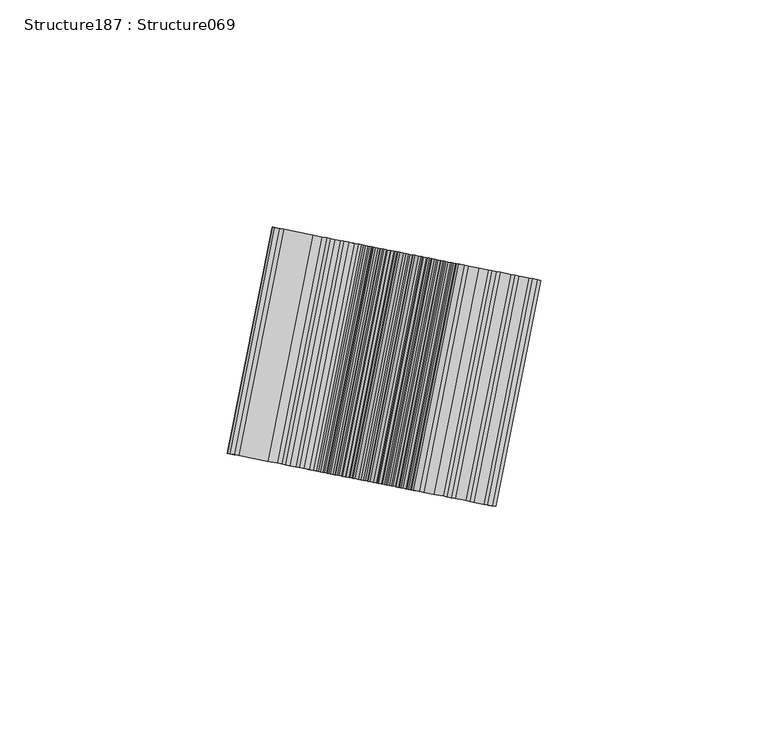
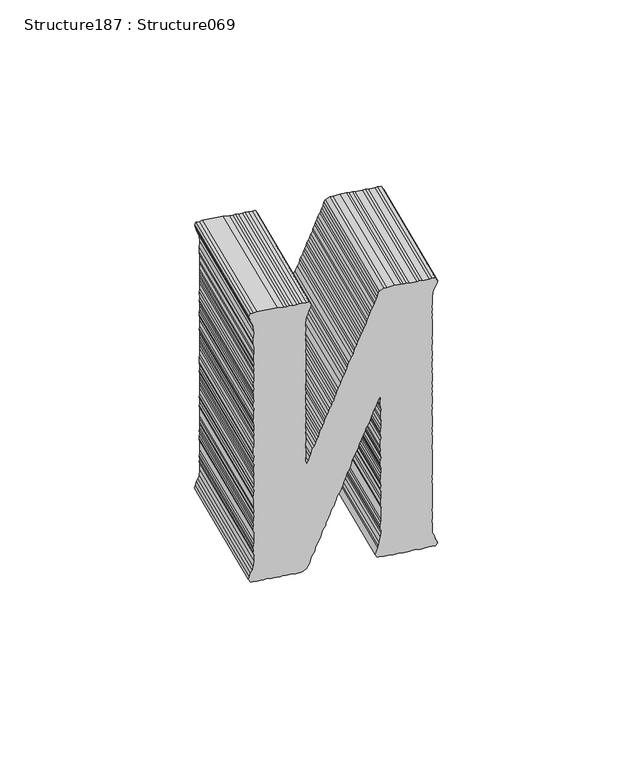
"""IFC4 building model written with IfcOpenShell, lengths in millimetres: proxy geometry, Structure187 : Structure069."""

import ifcopenshell
import ifcopenshell.guid

model = None  # the IFC model being written
_history = None  # IfcOwnerHistory: only IFC2X3 demands one
_inside = {}  # id of a spatial element -> (the spatial element, [elements in it])
_under = {}  # id of a project, library or spatial element -> (it, [spatial elements below it])
_declared = {}  # id of a project -> (the project, [libraries it declares])
_typed = {}  # id of a type object -> (the type object, [elements of that type])
_made_of = {}  # id of a material, layer set ... -> (it, [elements and type objects made of it])


def new_model(schema):
    """Start an empty IFC model of exactly this schema.

    Asked for "IFC4X3", IfcOpenShell would pick the latest addendum, in which some entities
    have other attributes; the version numbers below select the first issue.
    IFC2X3 requires an IfcOwnerHistory on every rooted entity: one is made here for all.
    """
    global model, _history
    if schema == "IFC4X3":
        model = ifcopenshell.file(schema_version=(4, 3, 0, 0))
    else:
        model = ifcopenshell.file(schema=schema)
    _inside.clear()
    _under.clear()
    _declared.clear()
    _typed.clear()
    _made_of.clear()
    _history = None
    if model.schema == "IFC2X3":
        org = make("IfcOrganization", Name="unknown")
        user = make(
            "IfcPersonAndOrganization",
            ThePerson=make("IfcPerson", FamilyName="unknown"),
            TheOrganization=org,
        )
        app = make(
            "IfcApplication",
            ApplicationDeveloper=org,
            Version="unknown",
            ApplicationFullName="unknown",
            ApplicationIdentifier="unknown",
        )
        _history = make(
            "IfcOwnerHistory",
            OwningUser=user,
            OwningApplication=app,
            ChangeAction="ADDED",
            CreationDate=0,
        )
    return model


def make(cls, **values):
    """One entity of the class cls with the attributes given. An attribute that is None is left unset."""
    return model.create_entity(
        cls, **{name: value for name, value in values.items() if value is not None}
    )


def rooted(cls, **values):
    """An entity with a GlobalId (a new one), such as an element, a storey or a relation."""
    return make(cls, GlobalId=ifcopenshell.guid.new(), OwnerHistory=_history, **values)


def si_unit(unit_type, name, prefix=None):
    """IfcSIUnit, for example si_unit("LENGTHUNIT", "METRE", prefix="MILLI")."""
    return make("IfcSIUnit", UnitType=unit_type, Prefix=prefix, Name=name)


def assignment(units):
    """IfcUnitAssignment: the units of a project."""
    return None if units is None else make("IfcUnitAssignment", Units=units)


def point(xyz):
    """IfcCartesianPoint."""
    return None if xyz is None else make("IfcCartesianPoint", Coordinates=xyz)


def direction(xyz):
    """IfcDirection."""
    return None if xyz is None else make("IfcDirection", DirectionRatios=xyz)


def frame(location, z_axis=None, x_axis=None):
    """IfcAxis2Placement3D, a coordinate frame: its origin and axes. An axis left out is left unset."""
    return make(
        "IfcAxis2Placement3D",
        Location=point(location),
        Axis=direction(z_axis),
        RefDirection=direction(x_axis),
    )


def origin():
    """The frame at (0, 0, 0) with its axes left unset."""
    return frame((0.0, 0.0, 0.0))


def place(relative_to, where):
    """IfcLocalPlacement: puts the frame where relative to a parent placement (None: the world)."""
    return make(
        "IfcLocalPlacement", PlacementRelTo=relative_to, RelativePlacement=where
    )


def context(
    kind, dimensions, precision=None, world=None, true_north=None, identifier=None
):
    """IfcGeometricRepresentationContext, for example the 3D "Model" context."""
    return make(
        "IfcGeometricRepresentationContext",
        ContextIdentifier=identifier,
        ContextType=kind,
        CoordinateSpaceDimension=dimensions,
        Precision=precision,
        WorldCoordinateSystem=world,
        TrueNorth=true_north,
    )


def project(units=None, contexts=None):
    """IfcProject with its units and contexts."""
    return rooted(
        "IfcProject",
        Name="project",
        RepresentationContexts=contexts,
        UnitsInContext=assignment(units),
    )


def spatial(cls, under=None, at=None, **own):
    """A site, building, storey or space (cls), placed at a placement, below another one or the project."""
    s = rooted(cls, ObjectPlacement=at, **own)
    if under is not None:
        _under.setdefault(under.id(), (under, []))[1].append(s)
    return s


def polyline(points):
    """IfcPolyline through the points."""
    return make("IfcPolyline", Points=[point(p) for p in points])


def outline(outer, holes=None, kind="AREA"):
    """IfcArbitraryClosedProfileDef: a profile drawn as a closed curve; with holes, ...WithVoids."""
    if holes is None:
        return make("IfcArbitraryClosedProfileDef", ProfileType=kind, OuterCurve=outer)
    return make(
        "IfcArbitraryProfileDefWithVoids",
        ProfileType=kind,
        OuterCurve=outer,
        InnerCurves=holes,
    )


def extrude(swept, where, along, depth):
    """IfcExtrudedAreaSolid: the profile swept, set in the frame where, extruded along a direction by depth."""
    return make(
        "IfcExtrudedAreaSolid",
        SweptArea=swept,
        Position=where,
        ExtrudedDirection=direction(along),
        Depth=depth,
    )


def shape(context_of_items, identifier, shape_type, items):
    """IfcShapeRepresentation: the items that make up one representation, for example the "Body"."""
    return make(
        "IfcShapeRepresentation",
        ContextOfItems=context_of_items,
        RepresentationIdentifier=identifier,
        RepresentationType=shape_type,
        Items=items,
    )


def source(mapping_origin, context_of_items, identifier, shape_type, items):
    """IfcRepresentationMap: a shape defined once, which mapped items show again and again."""
    return make(
        "IfcRepresentationMap",
        MappingOrigin=mapping_origin,
        MappedRepresentation=shape(context_of_items, identifier, shape_type, items),
    )


def transform(
    local_origin,
    x_axis=None,
    y_axis=None,
    z_axis=None,
    scale=None,
    scale2=None,
    scale3=None,
    uniform=True,
):
    """IfcCartesianTransformationOperator3D, or its non-uniform kind. x_axis, y_axis, z_axis: its Axis1, 2, 3."""
    if uniform:
        return make(
            "IfcCartesianTransformationOperator3D",
            Axis1=direction(x_axis),
            Axis2=direction(y_axis),
            LocalOrigin=point(local_origin),
            Scale=scale,
            Axis3=direction(z_axis),
        )
    return make(
        "IfcCartesianTransformationOperator3DnonUniform",
        Axis1=direction(x_axis),
        Axis2=direction(y_axis),
        LocalOrigin=point(local_origin),
        Scale=scale,
        Axis3=direction(z_axis),
        Scale2=scale2,
        Scale3=scale3,
    )


def mapped(mapping_source, mapping_target):
    """IfcMappedItem: shows the shape of a source again, moved by a transform."""
    return make(
        "IfcMappedItem", MappingSource=mapping_source, MappingTarget=mapping_target
    )


def made_of(thing, what):
    """Note that an element or type object is made of a material, layer set ...; save() writes the relation."""
    if what is not None:
        _made_of.setdefault(what.id(), (what, []))[1].append(thing)
    return thing


def element(
    cls,
    number,
    at=None,
    inside=None,
    cuts=None,
    type_object=None,
    material=None,
    context=None,
    identifier="Body",
    shape_type=None,
    held_by="IfcProductDefinitionShape",
    body=None,
    shapes=None,
    **own,
):
    """One element of the class cls, such as IfcWall. Its Tag is "e" and its number.

    at: its placement. inside: the storey or other place that contains it. cuts: it is an
    opening in that element (IfcRelVoidsElement). A single representation is given by context,
    identifier, shape_type and body (its items); several are given by shapes. held_by: the class
    of the entity that holds the representations. save() writes the other relations.
    """
    e = rooted(cls, Tag="e%d" % number, ObjectPlacement=at, **own)
    if body is not None:
        shapes = [shape(context, identifier, shape_type, body)]
    if shapes is not None:
        e.Representation = make(held_by, Representations=shapes)
    if inside is not None:
        _inside.setdefault(inside.id(), (inside, []))[1].append(e)
    if cuts is not None:
        rooted(
            "IfcRelVoidsElement", RelatingBuildingElement=cuts, RelatedOpeningElement=e
        )
    if type_object is not None:
        _typed.setdefault(type_object.id(), (type_object, []))[1].append(e)
    return made_of(e, material)


def aggregate(whole, parts):
    """IfcRelAggregates: a whole, such as a stair, and the parts it consists of."""
    return rooted("IfcRelAggregates", RelatingObject=whole, RelatedObjects=parts)


def save(model, path):
    """Write the relations noted so far, then the file.

    IfcRelAggregates (storeys below a building ...), IfcRelContainedInSpatialStructure (elements
    in a storey), IfcRelDefinesByType, IfcRelAssociatesMaterial and IfcRelDeclares: one each for
    every whole, place, type object, material and project.
    """
    for whole, parts in _under.values():
        aggregate(whole, parts)
    for where, things in _inside.values():
        rooted(
            "IfcRelContainedInSpatialStructure",
            RelatedElements=things,
            RelatingStructure=where,
        )
    for kind, things in _typed.values():
        rooted("IfcRelDefinesByType", RelatedObjects=things, RelatingType=kind)
    for what, things in _made_of.values():
        rooted("IfcRelAssociatesMaterial", RelatedObjects=things, RelatingMaterial=what)
    for by, libraries in _declared.values():
        rooted("IfcRelDeclares", RelatingContext=by, RelatedDefinitions=libraries)
    model.write(path)


def structure187_structure069_ac7f1eb3(model_context):
    return source(origin(), model_context, "Body", "SweptSolid", [
        extrude(outline(polyline([(1.8366799, 0.0), (3.1712942, 0.200391), (3.9678799, 0.2224656), (6.1339986, 0.7044792), (7.2010362, -0.1051671), (6.9235449, -1.1141613), (6.9103347, -2.1601811), (6.6008944, -4.347663), (6.6194392, -5.1387183), (6.4553745, -6.298517), (6.2008497, -7.1756413), (6.164673, -8.353531), (5.8912651, -10.2862941), (5.5038773, -11.150014), (5.322519, -12.4320637), (5.4724816, -13.2467403), (5.3278037, -14.2694911), (4.776401, -16.2926574), (4.4850018, -18.3526038), (3.4817959, -18.994451), (2.4116511, -18.1940678), (1.5481838, -17.8074344), (0.6787273, -17.4199537), (-0.4031239, -16.7429712), (-2.5708599, -16.3015649), (-3.6179366, -16.2882051), (-4.4817063, -15.9011696), (-5.5316583, -15.8827315), (-7.7145603, -15.5739391), (-8.6005421, -15.3185208), (-9.646971, -15.300581), (-13.7622837, -14.7184306), (-14.8072465, -14.7053698), (-15.8412712, -14.5590971), (-16.8492085, -14.2817554), (-18.0093595, -14.1176409), (-19.0175923, -13.844929), (-20.0827102, -13.9591049), (-20.8238767, -13.5894128), (-22.015121, -13.6857468), (-23.1509461, -13.3903142), (-24.0757719, -13.394248), (-27.2905847, -12.9394819), (-28.3002834, -12.661891), (-29.3265574, -12.5167147), (-30.11962, -12.5392877), (-31.3691672, -12.0976802), (-33.4665482, -12.0658325), (-34.4928222, -11.9206562), (-35.3742808, -11.6612062), (-36.5167429, -11.3695062), (-37.5628196, -11.3516163), (-38.4452783, -11.0966964), (-39.363467, -11.0968975), (-40.5405456, -11.0651477), (-42.5969688, -10.7742469), (-43.5925018, -10.3685722), (-44.619128, -10.2233461), (-45.6838937, -10.3375718), (-46.5473111, -9.9505861), (-47.870671, -10.0282311), (-48.6260031, -9.7866229), (-49.6713184, -9.7735123), (-50.7947394, -9.3497466), (-51.9916205, -9.4452833), (-52.7232746, -9.0769368), (-53.9145189, -9.1732708), (-54.7818118, -8.785737), (-56.1069332, -8.8631328), (-58.1672318, -8.5716838), (-59.0250123, -8.1854955), (-60.0943579, -8.2990733), (-61.0856633, -7.8939967), (-61.9896862, -7.766114), (-63.3091707, -7.8443072), (-64.300476, -7.4392306), (-65.1151027, -7.5888408), (-66.12304, -7.3114991), (-67.2591607, -7.0206962), (-68.4193117, -6.8565817), (-69.3565418, -6.9888485), (-70.5114082, -6.8254816), (-71.2486992, -6.4563377), (-72.4268915, -6.4197588), (-73.4774913, -6.4059007), (-74.6320055, -6.2425836), (-75.382053, -6.0017228), (-76.673615, -5.819019), (-77.7189303, -5.8059084), (-78.7109403, -5.4007321), (-79.7608922, -5.382294), (-80.6391233, -5.1279721), (-81.7077643, -5.2416496), (-82.829776, -4.8180833), (-83.6348904, -4.9690391), (-84.9045926, -4.6546682), (-85.695189, -4.6775901), (-88.0278455, -4.4773417), (-88.9646734, -4.6093061), (-90.2108917, -5.0917202), (-91.0201979, -5.2316617), (-92.1011932, -5.4733199), (-93.1586381, -4.5399739), (-93.1206999, -3.3623333), (-92.7520508, -2.6310813), (-92.4419626, -0.4390194), (-92.5752795, 0.4933282), (-92.1872438, 1.361628), (-91.8605099, 3.6713609), (-91.9924812, 4.6132208), (-91.587102, 5.604124), (-91.7377125, 6.4142205), (-91.4463133, 8.4741669), (-90.858928, 10.7516998), (-90.7315437, 11.6521997), (-89.7588844, 12.9570716), (-88.9368785, 13.2299759), (-87.6082839, 13.3065211), (-86.6587493, 13.5664163), (-85.7042326, 13.8259661), (-84.8931789, 13.9757224), (-83.7762507, 14.4713948), (-82.5614281, 14.6937624), (-81.6062067, 14.9532126), (-80.6633896, 15.0843297), (-79.4369103, 15.4297457), (-78.6501893, 15.4532158), (-77.5449109, 15.8208078), (-76.462154, 16.0622168), (-75.3815538, 16.2985405), (-74.534172, 16.7076455), (-73.5973441, 16.8396099), (-72.5103596, 17.0804208), (-71.687656, 17.3582574), (-70.4908177, 17.4484098), (-69.5003682, 17.9619738), (-68.5634905, 18.0942905), (-67.3684206, 18.1897241), (-66.2493787, 18.6850974), (-64.4672261, 19.2217862), (-63.5102931, 19.4806348), (-62.4663801, 19.4626916), (-61.3649772, 19.8308318), (-60.1522683, 20.0534986), (-59.1790557, 20.4401319), (-57.1602185, 20.8082206), (-55.3756066, 21.3495924), (-54.1625454, 21.5722092), (-53.227113, 21.694309), (-52.2712438, 21.9583392), (-51.0789855, 22.0491394), (-50.3414505, 22.6038709), (-49.2971852, 22.5858779), (-48.3063835, 23.0993921), (-47.1095521, 23.1945765), (-46.0035261, 23.5674531), (-45.0532801, 23.8222167), (-44.0981086, 24.0813145), (-43.3078576, 24.0992543), (-41.9481697, 24.436248), (-40.9757116, 24.8226287), (-40.0212378, 25.0767942), (-38.9505328, 25.1898204), (-37.8872262, 25.3038931), (-37.0641205, 25.5820322), (-35.977538, 25.8225407), (-34.8771851, 26.1857985), (-34.031515, 26.595505), (-32.0246798, 26.8355631), (-31.0761953, 27.0905759), (-29.7162049, 27.4271675), (-28.755699, 27.68587), (-29.9756481, 28.3773568), (-32.0655947, 28.4185743), (-34.1262456, 28.7100731), (-34.8632205, 29.0687508), (-36.0194961, 29.2323171), (-37.0630636, 29.2552425), (-38.22709, 29.4199052), (-39.2734691, 29.4381973), (-40.0065686, 29.7963268), (-41.0741166, 29.6929162), (-42.0672194, 30.0878256), (-43.0994827, 30.2338492), (-44.2889293, 30.1476823), (-45.1714379, 30.4022499), (-46.4404218, 30.7064571), (-47.2320888, 30.6937487), (-48.2724787, 30.7111936), (-49.4015725, 31.1253403), (-50.4469016, 31.1485149), (-51.4562342, 31.4159919), (-53.5165329, 31.7074409), (-54.5837286, 31.6039804), (-56.59923, 32.143518), (-57.3771267, 32.2535589), (-58.4411516, 32.1496499), (-59.7094377, 32.4587895), (-60.4996887, 32.4408498), (-61.5224396, 32.5855277), (-62.7787167, 33.0176657), (-63.5827382, 32.8769767), (-65.6433891, 33.1684755), (-66.9116752, 33.4776151), (-68.9719739, 33.7690641), (-69.8495432, 34.017902), (-70.9188528, 33.9147405), (-71.8010091, 34.1692583), (-72.9555232, 34.3325754), (-74.1022561, 34.619489), (-75.1479374, 34.6427134), (-75.9029036, 34.8742079), (-78.2468644, 34.9513581), (-79.2459565, 35.3471148), (-80.2718781, 35.4922413), (-82.2586151, 35.3840993), (-83.4695623, 35.1611835), (-84.4106677, 35.0294649), (-85.6374925, 34.6790667), (-86.7195018, 34.4429423), (-87.7897033, 35.2480053), (-87.5340788, 36.1303643), (-87.3520228, 37.4173463), (-87.3349372, 38.462818), (-86.9711776, 39.200152), (-86.7891714, 40.4867817), (-86.8981624, 41.5504475), (-86.5344027, 42.2877815), (-86.3890769, 43.3151123), (-86.3520443, 45.4110412), (-85.4425121, 51.8406667), (-85.0420721, 52.8372996), (-85.0228229, 53.8828246), (-83.9355358, 54.1232334), (-82.7042823, 53.5548448), (-81.9482524, 53.3181688), (-80.8667964, 52.6358518), (-79.8927349, 52.1088765), (-77.7419401, 51.5451693), (-75.6456589, 51.5080868), (-73.7185328, 51.2354763), (-72.7226045, 50.8351361), (-70.5397026, 50.5263436), (-69.7476901, 50.5440342), (-67.5556282, 50.233946), (-66.5508686, 49.9620848), (-65.5062512, 49.9440419), (-64.6184579, 49.6887268), (-63.5738403, 49.6706839), (-62.4316806, 49.3793861), (-60.3770189, 49.0887345), (-59.3066593, 49.1967785), (-57.2879802, 48.6517603), (-56.2200868, 48.7601532), (-55.0832117, 48.469603), (-54.1777794, 48.3415209), (-53.0409043, 48.0509707), (-52.2365374, 48.1966419), (-50.9442707, 48.0138384), (-50.0804581, 47.6321872), (-49.0358406, 47.6141443), (-46.8473017, 47.3045545), (-45.9252875, 47.303855), (-44.7887646, 47.0133546), (-44.0383716, 46.7774761), (-43.0064608, 46.6315024), (-41.8318415, 46.5950695), (-40.9493329, 46.3405019), (-39.7733044, 46.3038697), (-38.6307924, 46.0125221), (-36.576483, 45.7219203), (-35.6400005, 45.8489025), (-33.5797019, 45.5574535), (-32.7095476, 45.1749052), (-31.4109159, 45.1209296), (-30.6245403, 45.1394175), (-29.6282597, 44.7390274), (-28.5822329, 44.7207852), (-27.5538452, 44.5753099), (-26.2816836, 44.2656221), (-25.4953081, 44.2841101), (-24.2249081, 43.9746715), (-22.1663711, 43.6834717), (-21.2298885, 43.8104539), (-20.3657236, 43.4287528), (-19.059341, 43.3736808), (-18.0094388, 43.3548903), (-17.1329196, 43.10117), (-13.9177545, 42.646354), (-13.0299613, 42.3910388), (-11.8574559, 42.354905), (-11.1010736, 42.1181791), (-9.7968049, 42.0634061), (-9.0104293, 42.0818941), (-7.7421432, 41.7727545), (-6.8180151, 41.771756), (-5.7917412, 41.6265798), (-4.9275762, 41.2448787), (-1.7124111, 40.7900627), (-0.5342688, 40.7531315), (0.3782332, 40.7537777), (1.5263822, 40.4616327), (2.3127577, 40.4801206), (3.4348124, 40.0619386), (5.6233512, 39.7523488), (7.4599812, 39.7519964), (8.7945956, 39.9523874), (9.6459027, 40.3612965), (10.9833286, 40.5663207), (11.7940302, 40.7161269), (12.8430266, 39.7789449), (12.7156921, 38.8787974), (12.715498, 37.9552742), (12.4063016, 36.6916678), (12.2789172, 35.7911679), (11.982737, 34.6500582), (12.1340951, 33.8452462), (11.8234534, 32.5714229), (11.6606399, 30.4983179), (11.2725543, 29.6296657), (11.387232, 28.5655548), (10.9638616, 27.4474684), (10.8544685, 26.6741518), (10.9691462, 25.610041), (10.6771936, 24.4683332), (10.5498591, 23.5681856), (9.4634279, 22.4091361), (8.5124841, 22.1494402), (7.3948084, 21.6484832), (6.4706803, 21.6494817), (5.2621923, 21.4312489), (4.2826949, 21.040833), (3.3154715, 20.6533524), (2.1186401, 20.558168), (1.0144118, 20.1954584), (-0.8952764, 19.6768109), (-1.8472703, 19.4122325), (-2.6424604, 19.4000225), (-3.9777726, 19.1946992), (-4.8065152, 18.9173575), (-5.9244934, 18.4168026), (-6.8426322, 18.4169538), (-7.9493198, 18.0495611), (-8.9041889, 17.7900612), (-9.8713624, 17.4029328), (-11.0540779, 17.43548), (-11.8944274, 17.0354422), (-13.000101, 16.6625158), (-13.9147167, 16.6621686), (-15.0161129, 16.2889963), (-15.8236573, 16.1488056), (-16.9067168, 15.9077988), (-17.9021415, 15.3895482), (-19.94002, 14.8893937), (-20.9846376, 14.9074366), (-22.085738, 14.5388942), (-22.9183063, 14.2624529), (-24.2373886, 14.1845622), (-26.0371803, 13.5206404), (-27.1258766, 13.2804309), (-28.0443677, 13.280632), (-29.2528558, 13.0623992), (-30.0797871, 12.7851607), (-31.181233, 12.4116361), (-31.990173, 12.2615808), (-33.2413305, 11.7848964), (-34.2873573, 11.8031386), (-35.3923332, 11.4351444), (-36.3235242, 11.3023826), (-37.429148, 10.9298085), (-39.4663786, 10.4342339), (-40.4032065, 10.3022696), (-41.2615472, 9.7750486), (-42.2223557, 9.5167482), (-43.3040488, 9.2701577), (-44.3722945, 9.1618146), (-45.1773591, 9.0112111), (-46.3854949, 8.7929286), (-47.5112736, 8.2931178), (-48.4484538, 8.1612033), (-49.2753851, 7.8839647), (-50.3573944, 7.6478403), (-51.4623703, 7.2798462), (-50.4487962, 7.001707), (-49.5334827, 7.0069865), (-48.2419206, 6.8242826), (-47.3601098, 6.5647826), (-46.3514748, 6.2923732), (-45.4333359, 6.292222), (-43.3726851, 6.0007232), (-42.104399, 5.6915836), (-40.3037515, 5.4368647), (-38.9977213, 5.3818425), (-38.2106479, 5.4052629), (-37.1970738, 5.1271237), (-36.060551, 4.8366233), (-34.9954828, 4.9504469), (-32.8090579, 4.6411561), (-31.7954837, 4.3630169), (-30.8766472, 4.3677981), (-29.740822, 4.0723653), (-28.8526765, 3.8170003), (-27.7897223, 3.9311229), (-26.6330943, 3.7675068), (-25.7477604, 3.5075084), (-24.8694795, 3.2535388), (-23.8372163, 3.1075153), (-22.9190774, 3.1073641), (-21.6324477, 2.9253579), (-20.5857232, 2.9120481), (-19.577786, 2.6347063), (-18.6899929, 2.3793911), (-17.6249247, 2.4932147), (-16.5070909, 2.0705987), (-14.4485539, 1.7793989), (-13.5300626, 1.7791978), (-11.469764, 1.4877488), (-10.5876078, 1.233231), (-6.2122917, 0.6143006), (-5.2997897, 0.6149467), (-4.1149604, 0.5821006), (-3.2204497, 0.4555635), (-2.3513456, 0.0681327), (-1.3247193, -0.0770935), (0.0, 0.0), (1.8366799, 0.0)])), frame((-2680.5507815, 235000.456428, 393.6733864), z_axis=(0.19466222296394126, 0.9808703374813295, 0.0), x_axis=(-0.13738573096273865, 0.027265389492153222, -0.990142292533591)), (0.0, 0.0, 1.0), 50.8),
    ])


if __name__ == "__main__":
    model = new_model("IFC4")
    model_context = context("Model", 3, world=origin())
    ifc_project = project(units=[si_unit("LENGTHUNIT", "METRE", prefix="MILLI")], contexts=[model_context])
    site = spatial("IfcSite", under=ifc_project)
    building = spatial("IfcBuilding", under=site)
    placement = place(None, origin())
    structure187_structure069_shape = structure187_structure069_ac7f1eb3(model_context)
    element("IfcBuildingElementProxy", 1, Name="Structure187 : Structure069", ObjectType="Structure187 : Structure069", at=placement, inside=building, context=model_context, shape_type="MappedRepresentation", body=[
        mapped(structure187_structure069_shape, transform((0.0, 0.0, 0.0), x_axis=(1.0, 0.0, 0.0), y_axis=(0.0, 1.0, 0.0), z_axis=(0.0, 0.0, 1.0))),
    ])
    save(model, "model.ifc")

# Revit data of these elements
# Type "Structure187 : Structure069"
#   NameOverride = "Structure069"
# Element 1 (IfcBuildingElementProxy, "Structure187 : Structure069")
#   Materials on its faces: "BRUSHED ALUMINUM LETTERING"
# Materials
#   "BRUSHED ALUMINUM LETTERING": class "Unassigned", colour RGB 169 181 186, transparency 0, Cost = 0
